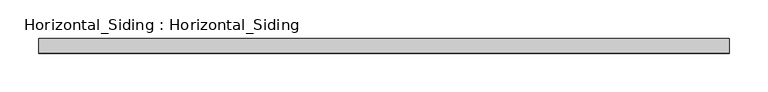
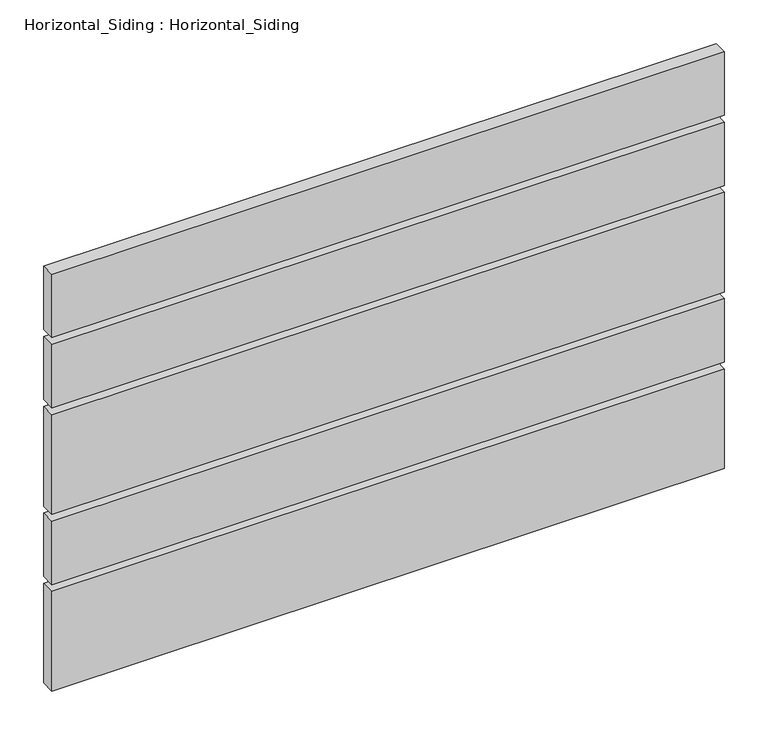
"""IFC4 building model written with IfcOpenShell, lengths in millimetres: plate geometry, Horizontal_Siding : Horizontal_Siding."""

from ifc_helpers import new_model, si_unit, frame, origin, place, context, project, spatial, polyline, outline, extrude, source, transform, mapped, element, save


def horizontal_siding_horizontal_siding_9efb88d0(model_context):
    return source(origin(), model_context, "Body", "SweptSolid", [
        extrude(outline(polyline([(445.6444437, -19.05), (-445.6444437, -19.05), (-445.6444437, 0.0), (445.6444437, 0.0), (445.6444437, -19.05)])), frame((0.0, 0.0, 9.525), z_axis=(0.0, 0.0, 1.0), x_axis=(1.0, 0.0, 0.0)), (0.0, 0.0, 1.0), 139.7),
        extrude(outline(polyline([(445.6444437, -19.05), (-445.6444437, -19.05), (-445.6444437, 0.0), (445.6444437, 0.0), (445.6444437, -19.05)])), frame((0.0, 0.0, 158.75), z_axis=(0.0, 0.0, 1.0), x_axis=(1.0, 0.0, 0.0)), (0.0, 0.0, 1.0), 88.9),
        extrude(outline(polyline([(445.6444437, -19.05), (-445.6444437, -19.05), (-445.6444437, 0.0), (445.6444437, 0.0), (445.6444437, -19.05)])), frame((0.0, 0.0, 257.175), z_axis=(0.0, 0.0, 1.0), x_axis=(1.0, 0.0, 0.0)), (0.0, 0.0, 1.0), 139.7),
        extrude(outline(polyline([(445.6444437, -19.05), (-445.6444437, -19.05), (-445.6444437, 0.0), (445.6444437, 0.0), (445.6444437, -19.05)])), frame((0.0, 0.0, 406.4), z_axis=(0.0, 0.0, 1.0), x_axis=(1.0, 0.0, 0.0)), (0.0, 0.0, 1.0), 88.9),
        extrude(outline(polyline([(445.6444437, -19.05), (-445.6444437, -19.05), (-445.6444437, 0.0), (445.6444437, 0.0), (445.6444437, -19.05)])), frame((0.0, 0.0, 504.825), z_axis=(0.0, 0.0, 1.0), x_axis=(1.0, 0.0, 0.0)), (0.0, 0.0, 1.0), 88.9),
    ])


if __name__ == "__main__":
    model = new_model("IFC4")
    model_context = context("Model", 3, world=origin())
    ifc_project = project(units=[si_unit("LENGTHUNIT", "METRE", prefix="MILLI")], contexts=[model_context])
    site = spatial("IfcSite", under=ifc_project)
    building = spatial("IfcBuilding", under=site)
    placement = place(None, origin())
    horizontal_siding_horizontal_siding_shape = horizontal_siding_horizontal_siding_9efb88d0(model_context)
    element("IfcPlate", 1, ObjectType="Horizontal_Siding : Horizontal_Siding", at=placement, inside=building, context=model_context, shape_type="MappedRepresentation", body=[
        mapped(horizontal_siding_horizontal_siding_shape, transform((0.0, 0.0, 0.0), x_axis=(1.0, 0.0, 0.0), y_axis=(0.0, 1.0, 0.0), z_axis=(0.0, 0.0, 1.0))),
    ])
    save(model, "model.ifc")

# Revit data of these elements
# Type "Horizontal_Siding : Horizontal_Siding"
#   Analytic Construction = "<None>"
#   extend = 0' - 2 3/4"
#   Width_2 = 0' - 3 1/2"
#   Width_1 = 0' - 5 1/2"
#   Gap = 0' - 0 3/8"
#   Plank Material = SLOTTED WOOD FENCE (THERMALLY MODIFIED WOOD: ARBOR WOOD)\n(EXTERIOR STAIN : PENOFIN VERDE EXT. STAIN - COLOR: CEDAR)
# Element 1 (IfcPlate, "Horizontal_Siding : Horizontal_Siding")
#   Materials on its faces: "SLOTTED WOOD FENCE (THERMALLY MODIFIED WOOD: ARBOR WOOD)\n(EXTERIOR STAIN : PENOFIN VERDE EXT. STAIN - COLOR: CEDAR)"
# Materials
#   "SLOTTED WOOD FENCE (THERMALLY MODIFIED WOOD: ARBOR WOOD)\n(EXTERIOR STAIN : PENOFIN VERDE EXT. STAIN - COLOR: CEDAR)": class "Wood", colour RGB 164 134 123, transparency 0, Description = "Pinus Echinata", Cost = 0
